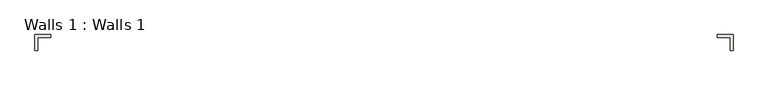
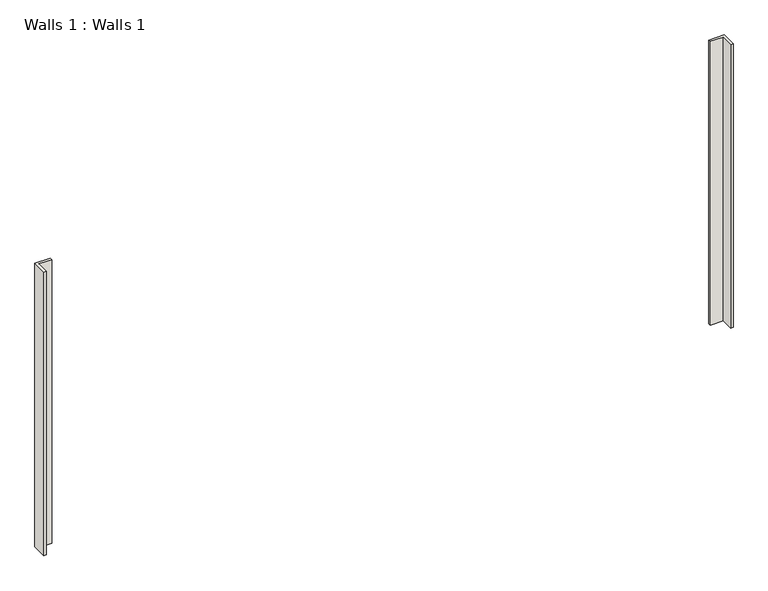
"""IFC4 building model written with IfcOpenShell, lengths in millimetres: wall geometry, Walls 1 : Walls 1."""

from ifc_helpers import new_model, si_unit, frame, origin, place, context, project, spatial, polyline, outline, extrude, source, transform, mapped, element, save


def walls_1_walls_1_6286a9b3(model_context):
    return source(origin(), model_context, "Body", "SweptSolid", [
        extrude(outline(polyline([(25914.0402986, -1873.6830088), (25787.0402986, -1873.6830088), (25787.0402986, -2000.6830088), (25761.6402986, -2000.6830088), (25761.6402986, -1848.2830088), (25914.0402986, -1848.2830088), (25914.0402986, -1873.6830088)])), frame((0.0, 0.0, 3657.6), z_axis=(0.0, 0.0, 1.0), x_axis=(1.0, 0.0, 0.0)), (0.0, 0.0, 1.0), 2966.3300391),
        extrude(outline(polyline([(32425.9652986, -1873.6830088), (32425.9652986, -1848.2830088), (32578.3652986, -1848.2830088), (32578.3652986, -2000.6830088), (32552.9652986, -2000.6830088), (32552.9652986, -1873.6830088), (32425.9652986, -1873.6830088)])), frame((0.0, 0.0, 3657.6), z_axis=(0.0, 0.0, 1.0), x_axis=(1.0, 0.0, 0.0)), (0.0, 0.0, 1.0), 2966.3300391),
    ])


if __name__ == "__main__":
    model = new_model("IFC4")
    model_context = context("Model", 3, world=origin())
    ifc_project = project(units=[si_unit("LENGTHUNIT", "METRE", prefix="MILLI")], contexts=[model_context])
    site = spatial("IfcSite", under=ifc_project)
    building = spatial("IfcBuilding", under=site)
    placement = place(None, origin())
    walls_1_walls_1_shape = walls_1_walls_1_6286a9b3(model_context)
    element("IfcWall", 1, ObjectType="Walls 1 : Walls 1", at=placement, inside=building, context=model_context, shape_type="MappedRepresentation", body=[
        mapped(walls_1_walls_1_shape, transform((0.0, 0.0, 0.0), x_axis=(1.0, 0.0, 0.0), y_axis=(0.0, 1.0, 0.0), z_axis=(0.0, 0.0, 1.0))),
    ])
    save(model, "model.ifc")

# Revit data of these elements
# Element 1 (IfcWall, "Walls 1 : Walls 1")
#   Materials on its faces: "Trim"
# Materials
#   "Trim": class "Wood", colour RGB 250 251 245, transparency 0, Cost = 0
